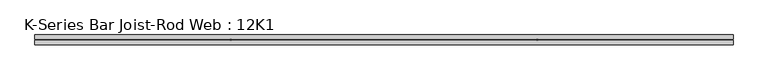
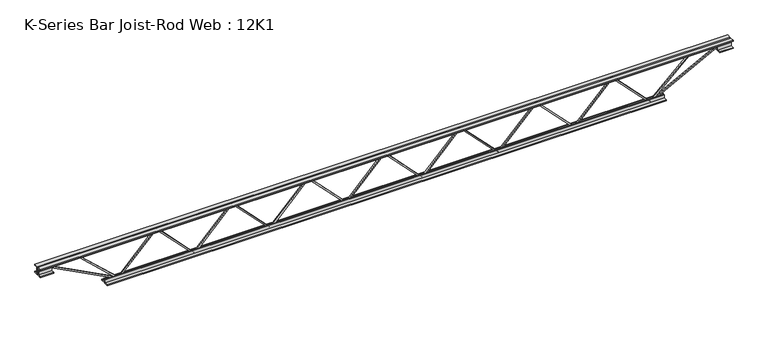
"""IFC4 building model written with IfcOpenShell, lengths in millimetres: beam geometry, K-Series Bar Joist-Rod Web : 12K1."""

from ifc_helpers import new_model, si_unit, frame, origin, place, context, project, spatial, polyline, outline, extrude, source, transform, mapped, element, save


def k_series_bar_joist_rod_web_12k1_8968bb53(model_context):
    return source(origin(), model_context, "Body", "SweptSolid", [
        extrude(outline(polyline([(-141.2875, 866.0946429), (-150.8125, 866.0946429), (-150.8125, 871.2898582), (141.2875, 1153.6380724), (141.2875, 1155.9476418), (-150.8125, 1438.2958561), (-150.8125, 1443.4910714), (-141.2875, 1443.4910714), (-141.2875, 1442.3362867), (150.8125, 1159.9880724), (150.8125, 1149.5976418), (-141.2875, 867.2494276), (-141.2875, 866.0946429)])), frame((0.0, -4.7625, 0.0), z_axis=(0.0, 1.0, 0.0), x_axis=(0.0, 0.0, 1.0)), (0.0, 0.0, 1.0), 9.525),
        extrude(outline(polyline([(-141.2875, 288.6982143), (-150.8125, 288.6982143), (-150.8125, 293.8934296), (141.2875, 576.2416439), (141.2875, 578.5512133), (-150.8125, 860.8994276), (-150.8125, 866.0946429), (-141.2875, 866.0946429), (-141.2875, 864.9398582), (150.8125, 582.5916439), (150.8125, 572.2012133), (-141.2875, 289.852999), (-141.2875, 288.6982143)])), frame((0.0, -4.7625, 0.0), z_axis=(0.0, 1.0, 0.0), x_axis=(0.0, 0.0, 1.0)), (0.0, 0.0, 1.0), 9.525),
        extrude(outline(polyline([(-141.2875, -288.6982143), (-150.8125, -288.6982143), (-150.8125, -283.502999), (141.2875, -1.1547847), (141.2875, 1.1547847), (-150.8125, 283.502999), (-150.8125, 288.6982143), (-141.2875, 288.6982143), (-141.2875, 287.5434296), (150.8125, 5.1952153), (150.8125, -5.1952153), (-141.2875, -287.5434296), (-141.2875, -288.6982143)])), frame((0.0, -4.7625, 0.0), z_axis=(0.0, 1.0, 0.0), x_axis=(0.0, 0.0, 1.0)), (0.0, 0.0, 1.0), 9.525),
        extrude(outline(polyline([(-141.2875, -866.0946429), (-150.8125, -866.0946429), (-150.8125, -860.8994276), (141.2875, -578.5512133), (141.2875, -576.2416439), (-150.8125, -293.8934296), (-150.8125, -288.6982143), (-141.2875, -288.6982143), (-141.2875, -289.852999), (150.8125, -572.2012133), (150.8125, -582.5916439), (-141.2875, -864.9398582), (-141.2875, -866.0946429)])), frame((0.0, -4.7625, 0.0), z_axis=(0.0, 1.0, 0.0), x_axis=(0.0, 0.0, 1.0)), (0.0, 0.0, 1.0), 9.525),
        extrude(outline(polyline([(-141.2875, -1443.4910714), (-150.8125, -1443.4910714), (-150.8125, -1438.2958561), (141.2875, -1155.9476418), (141.2875, -1153.6380724), (-150.8125, -871.2898582), (-150.8125, -866.0946429), (-141.2875, -866.0946429), (-141.2875, -867.2494276), (150.8125, -1149.5976418), (150.8125, -1159.9880724), (-141.2875, -1442.3362867), (-141.2875, -1443.4910714)])), frame((0.0, -4.7625, 0.0), z_axis=(0.0, 1.0, 0.0), x_axis=(0.0, 0.0, 1.0)), (0.0, 0.0, 1.0), 9.525),
        extrude(outline(polyline([(-141.2875, 1443.4910714), (-150.8125, 1443.4910714), (-150.8125, 1448.6862867), (141.2875, 1731.034501), (141.2875, 1733.3440704), (-150.8125, 2015.6922847), (-150.8125, 2020.8875), (-141.2875, 2020.8875), (-141.2875, 2019.7327153), (150.8125, 1737.384501), (150.8125, 1726.9940704), (-141.2875, 1444.6458561), (-141.2875, 1443.4910714)])), frame((0.0, -4.7625, 0.0), z_axis=(0.0, 1.0, 0.0), x_axis=(0.0, 0.0, 1.0)), (0.0, 0.0, 1.0), 9.525),
        extrude(outline(polyline([(-141.2875, -2020.8875), (-150.8125, -2020.8875), (-150.8125, -2015.6922847), (141.2875, -1733.3440704), (141.2875, -1731.034501), (-150.8125, -1448.6862867), (-150.8125, -1443.4910714), (-141.2875, -1443.4910714), (-141.2875, -1444.6458561), (150.8125, -1726.9940704), (150.8125, -1737.384501), (-141.2875, -2019.7327153), (-141.2875, -2020.8875)])), frame((0.0, -4.7625, 0.0), z_axis=(0.0, 1.0, 0.0), x_axis=(0.0, 0.0, 1.0)), (0.0, 0.0, 1.0), 9.525),
        extrude(outline(polyline([(4.7625, 152.4), (36.5125, 152.4), (36.5125, 146.05), (11.1125, 146.05), (11.1125, 120.65), (4.7625, 120.65), (4.7625, 152.4)])), frame((-2630.4875, 0.0, 0.0), z_axis=(1.0, 0.0, 0.0), x_axis=(0.0, 1.0, 0.0)), (0.0, 0.0, 1.0), 5260.975),
        extrude(outline(polyline([(-4.7625, 152.4), (-4.7625, 120.65), (-11.1125, 120.65), (-11.1125, 146.05), (-36.5125, 146.05), (-36.5125, 152.4), (-4.7625, 152.4)])), frame((-2630.4875, 0.0, 0.0), z_axis=(1.0, 0.0, 0.0), x_axis=(0.0, 1.0, 0.0)), (0.0, 0.0, 1.0), 5260.975),
        extrude(outline(polyline([(-4.7625, 88.9), (-36.5125, 88.9), (-36.5125, 95.25), (-11.1125, 95.25), (-11.1125, 120.65), (-4.7625, 120.65), (-4.7625, 88.9)])), frame((-2630.4875, 0.0, 0.0), z_axis=(1.0, 0.0, 0.0), x_axis=(0.0, 1.0, 0.0)), (0.0, 0.0, 1.0), 101.6),
        extrude(outline(polyline([(36.5125, 88.9), (4.7625, 88.9), (4.7625, 120.65), (11.1125, 120.65), (11.1125, 95.25), (36.5125, 95.25), (36.5125, 88.9)])), frame((-2630.4875, 0.0, 0.0), z_axis=(1.0, 0.0, 0.0), x_axis=(0.0, 1.0, 0.0)), (0.0, 0.0, 1.0), 101.6),
        extrude(outline(polyline([(4.7625, 88.9), (4.7625, 120.65), (11.1125, 120.65), (11.1125, 95.25), (36.5125, 95.25), (36.5125, 88.9), (4.7625, 88.9)])), frame((2528.8875, 0.0, 0.0), z_axis=(1.0, 0.0, 0.0), x_axis=(0.0, 1.0, 0.0)), (0.0, 0.0, 1.0), 101.6),
        extrude(outline(polyline([(-4.7625, 88.9), (-36.5125, 88.9), (-36.5125, 95.25), (-11.1125, 95.25), (-11.1125, 120.65), (-4.7625, 120.65), (-4.7625, 88.9)])), frame((2528.8875, 0.0, 0.0), z_axis=(1.0, 0.0, 0.0), x_axis=(0.0, 1.0, 0.0)), (0.0, 0.0, 1.0), 101.6),
        extrude(outline(polyline([(4.7625, -152.4), (4.7625, -120.65), (11.1125, -120.65), (11.1125, -146.05), (36.5125, -146.05), (36.5125, -152.4), (4.7625, -152.4)])), frame((-2122.4875, 0.0, 0.0), z_axis=(1.0, 0.0, 0.0), x_axis=(0.0, 1.0, 0.0)), (0.0, 0.0, 1.0), 4244.975),
        extrude(outline(polyline([(-4.7625, -152.4), (-36.5125, -152.4), (-36.5125, -146.05), (-11.1125, -146.05), (-11.1125, -120.65), (-4.7625, -120.65), (-4.7625, -152.4)])), frame((-2122.4875, 0.0, 0.0), z_axis=(1.0, 0.0, 0.0), x_axis=(0.0, 1.0, 0.0)), (0.0, 0.0, 1.0), 4244.975),
        extrude(outline(polyline([(0.0, -9.525), (0.0, 0.0), (573.7533355, 0.0), (573.7533355, -9.525), (0.0, -9.525)])), frame((-2531.1012714, 4.7625, 116.4332925), z_axis=(0.4648338989895136, 0.0, 0.8853979028381571), x_axis=(0.8853979028381571, 0.0, -0.4648338989895136)), (0.0, 0.0, 1.0), 9.525),
        extrude(outline(polyline([(0.0, -9.525), (0.0, 0.0), (393.0337758, 0.0), (393.0337758, -9.525), (0.0, -9.525)])), frame((-2312.8173927, 4.7625, 117.1517631), z_axis=(0.6785676356860265, 0.0, 0.7345379253649712), x_axis=(0.7345379253649712, 0.0, -0.6785676356860265)), (0.0, 0.0, 1.0), 9.525),
        extrude(outline(polyline([(0.0, -9.525), (0.0, 0.0), (573.7533355, 0.0), (573.7533355, -9.525), (0.0, -9.525)])), frame((2531.1012714, -4.7625, 116.4332925), z_axis=(-0.4648338989894956, 0.0, 0.8853979028381666), x_axis=(-0.8853979028381666, 0.0, -0.4648338989894956)), (0.0, 0.0, 1.0), 9.525),
        extrude(outline(polyline([(0.0, -9.525), (0.0, 0.0), (393.0337758, 0.0), (393.0337758, -9.525), (0.0, -9.525)])), frame((2312.8173927, -4.7625, 117.1517631), z_axis=(-0.6785676356860202, 0.0, 0.7345379253649771), x_axis=(-0.7345379253649771, 0.0, -0.6785676356860202)), (0.0, 0.0, 1.0), 9.525),
    ])


if __name__ == "__main__":
    model = new_model("IFC4")
    model_context = context("Model", 3, world=origin())
    ifc_project = project(units=[si_unit("LENGTHUNIT", "METRE", prefix="MILLI")], contexts=[model_context])
    site = spatial("IfcSite", under=ifc_project)
    building = spatial("IfcBuilding", under=site)
    placement = place(None, origin())
    k_series_bar_joist_rod_web_12k1_shape = k_series_bar_joist_rod_web_12k1_8968bb53(model_context)
    element("IfcBeam", 1, ObjectType="K-Series Bar Joist-Rod Web : 12K1", at=placement, inside=building, context=model_context, shape_type="MappedRepresentation", body=[
        mapped(k_series_bar_joist_rod_web_12k1_shape, transform((0.0, 0.0, 0.0), x_axis=(1.0, 0.0, 0.0), y_axis=(0.0, 1.0, 0.0), z_axis=(0.0, 0.0, 1.0))),
    ])
    save(model, "model.ifc")

# Revit data of these elements
# Type "K-Series Bar Joist-Rod Web : 12K1"
#   Assembly Code = "B1010350"
#   Wt = 5
#   Web Thickness = 9.525 mm
#   Start Offset [instance default] = 0 mm
#   Start Extension [instance default] = 0 mm
#   Seat Length = 101.6 mm
#   Seat Depth = 63.5 mm
#   PanelArrayLength [instance default] = 6096 mm
#   Panel [instance default] = 609.6 mm
#   End Offset [instance default] = 0 mm
#   End Extension [instance default] = 0 mm
#   End Panel = 609.6 mm
#   Cord Leg = 31.75 mm
#   Chord Thickness = 6.35 mm
#   Length [instance default] = 7315.2 mm
#   Depth = 304.8 mm
#   PanelArrayNum [instance default] = 10
#   Structural Material = Steel ASTM A500, Grade C, Round
# Element 1 (IfcBeam, "K-Series Bar Joist-Rod Web : 12K1")
#   PanelArrayLength = 4041.775 mm
#   Panel = 577.396 mm
#   PanelArrayNum = 7
#   Materials on its faces: "Steel ASTM A500, Grade C, Round"
# Materials
#   "Steel ASTM A500, Grade C, Round": class "Metal", colour RGB 202 101 0, transparency 0, Description = "Carbon steel", Cost = 0
